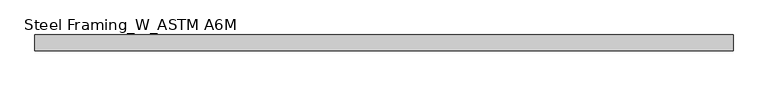
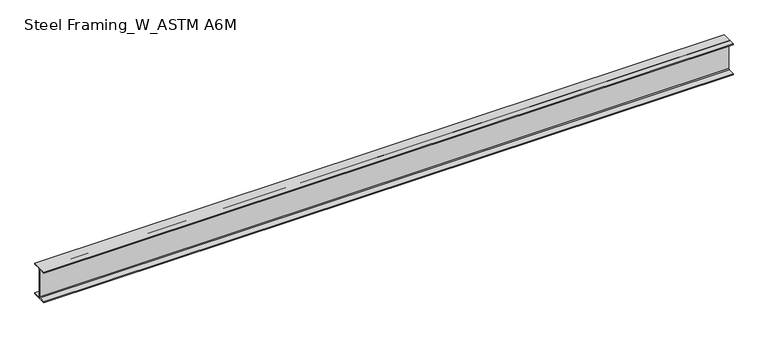
"""IFC4 building model written with IfcOpenShell, lengths in millimetres: beam geometry, Steel Framing_W_ASTM A6M : H_SB_AR_S02_W360x51_RG1."""

from ifc_helpers import new_model, si_unit, point, frame, frame_2d, origin, place, context, project, spatial, polyline, circle_curve, trimmed, segment, composite_curve, outline, extrude, source, transform, mapped, element, save


def steel_framing_w_astm_a6m_20e71bf1(model_context):
    return source(origin(), model_context, "Body", "SweptSolid", [
        extrude(outline(composite_curve([segment(polyline([(85.5, -166.4), (85.5, -178.0), (-85.5, -178.0), (-85.5, -166.4), (-13.72, -166.4)]), True, "CONTINUOUS"), segment(trimmed(circle_curve(frame_2d((-13.72, -156.3)), 10.1), [point((-13.72, -166.4))], [point((-3.62, -156.3))], True, "CARTESIAN"), True, "CONTINUOUS"), segment(polyline([(-3.62, -156.3), (-3.62, 156.3)]), True, "CONTINUOUS"), segment(trimmed(circle_curve(frame_2d((-13.72, 156.3)), 10.1), [point((-3.62, 156.3))], [point((-13.72, 166.4))], True, "CARTESIAN"), True, "CONTINUOUS"), segment(polyline([(-13.72, 166.4), (-85.5, 166.4), (-85.5, 178.0), (85.5, 178.0), (85.5, 166.4), (13.72, 166.4)]), True, "CONTINUOUS"), segment(trimmed(circle_curve(frame_2d((13.72, 156.3)), 10.1), [point((13.72, 166.4))], [point((3.62, 156.3))], True, "CARTESIAN"), True, "CONTINUOUS"), segment(polyline([(3.62, 156.3), (3.62, -156.3)]), True, "CONTINUOUS"), segment(trimmed(circle_curve(frame_2d((13.72, -156.3)), 10.1), [point((3.62, -156.3))], [point((13.72, -166.4))], True, "CARTESIAN"), True, "CONTINUOUS"), segment(polyline([(13.72, -166.4), (85.5, -166.4)]), True, "CONTINUOUS")], self_intersect=False)), frame((-3748.7, 0.0, 0.0), z_axis=(1.0, 0.0, 0.0), x_axis=(0.0, 1.0, 0.0)), (0.0, 0.0, 1.0), 7566.7),
    ])


if __name__ == "__main__":
    model = new_model("IFC4")
    model_context = context("Model", 3, world=origin())
    ifc_project = project(units=[si_unit("LENGTHUNIT", "METRE", prefix="MILLI")], contexts=[model_context])
    site = spatial("IfcSite", under=ifc_project)
    building = spatial("IfcBuilding", under=site)
    placement = place(None, origin())
    steel_framing_w_astm_a6m_shape = steel_framing_w_astm_a6m_20e71bf1(model_context)
    element("IfcBeam", 1, ObjectType="Steel Framing_W_ASTM A6M : H_SB_AR_S02_W360x51_RG1", at=placement, inside=building, context=model_context, shape_type="MappedRepresentation", body=[
        mapped(steel_framing_w_astm_a6m_shape, transform((0.0, 0.0, 0.0), x_axis=(1.0, 0.0, 0.0), y_axis=(0.0, 1.0, 0.0), z_axis=(0.0, 0.0, 1.0))),
    ])
    save(model, "model.ifc")

# Revit data of these elements
# Type "Steel Framing_W_ASTM A6M : H_SB_AR_S02_W360x51_RG1"
#   Section Name Key = "W14x34"
#   Width = 17.1 cm
#   Web Thickness = 0.724 cm
#   Web Fillet = 1.01 cm
#   Warping Constant = 287000.0 cm⁶
#   Torsional Moment of Inertia = 23.70 cm⁴
#   Section Area = 64.5 cm²
#   Plastic Modulus weak axis = 174.0 cm³
#   Plastic Modulus strong axis = 895.0 cm³
#   Perimeter = 1.36 m²/m
#   Nominal Weight = 51.00 kgf/m
#   Moment of Inertia weak axis = 970.00 cm⁴
#   Moment of Inertia strong axis = 14200.00 cm⁴
#   Height = 35.6 cm
#   Flange Thickness = 1.16 cm
#   Elastic Modulus weak axis = 113.0 cm³
#   Elastic Modulus strong axis = 796.0 cm³
#   Centroid Vertical = 17.8 cm
#   Centroid Horizontal = 8.55 cm
#   Length [instance default] = 1500 mm
#   Structural Material [instance default] = Steel, 45-345
#   Bolt Spacing = 0
#   Assembly Code = ""
# Element 1 (IfcBeam, "Steel Framing_W_ASTM A6M : H_SB_AR_S02_W360x51_RG1")
#   Materials on its faces: "Steel, 45-345"
# Materials
#   "Steel, 45-345": class "Metal", colour RGB 189 187 185, transparency 0, Description = "Steel 345 MPa", Cost = 0
